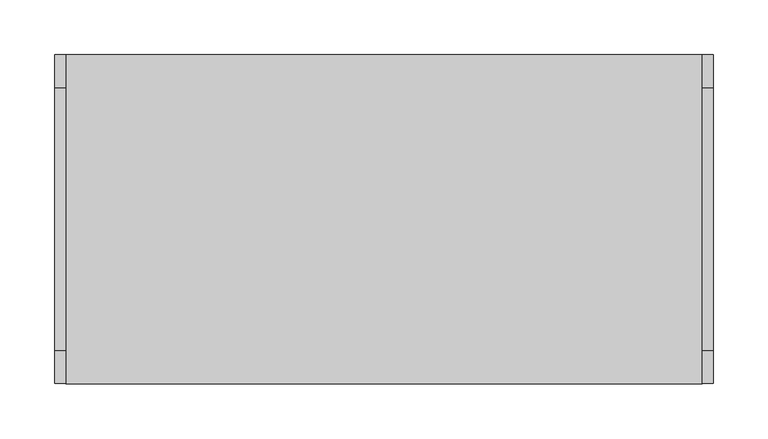
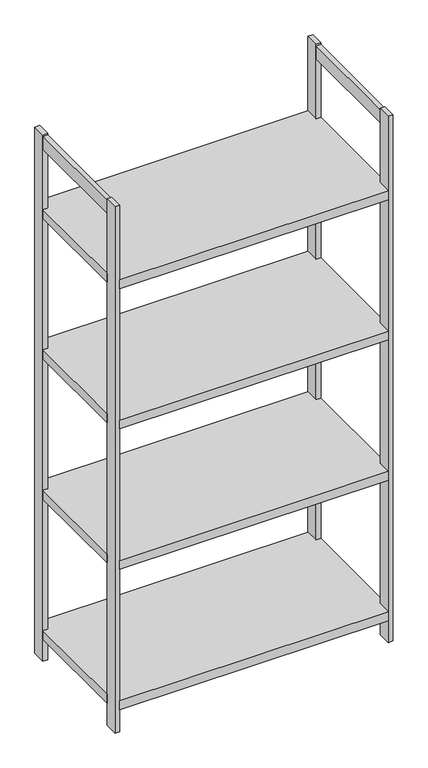
"""IFC4 building model written with IfcOpenShell, lengths in millimetres: furniture geometry, GEL-Shelf-一般オフィス棚 : GEL-Shelf-一般オフィス棚."""

import ifcopenshell
import ifcopenshell.guid

model = None  # the IFC model being written
_history = None  # IfcOwnerHistory: only IFC2X3 demands one
_inside = {}  # id of a spatial element -> (the spatial element, [elements in it])
_under = {}  # id of a project, library or spatial element -> (it, [spatial elements below it])
_declared = {}  # id of a project -> (the project, [libraries it declares])
_typed = {}  # id of a type object -> (the type object, [elements of that type])
_made_of = {}  # id of a material, layer set ... -> (it, [elements and type objects made of it])


def new_model(schema):
    """Start an empty IFC model of exactly this schema.

    Asked for "IFC4X3", IfcOpenShell would pick the latest addendum, in which some entities
    have other attributes; the version numbers below select the first issue.
    IFC2X3 requires an IfcOwnerHistory on every rooted entity: one is made here for all.
    """
    global model, _history
    if schema == "IFC4X3":
        model = ifcopenshell.file(schema_version=(4, 3, 0, 0))
    else:
        model = ifcopenshell.file(schema=schema)
    _inside.clear()
    _under.clear()
    _declared.clear()
    _typed.clear()
    _made_of.clear()
    _history = None
    if model.schema == "IFC2X3":
        org = make("IfcOrganization", Name="unknown")
        user = make(
            "IfcPersonAndOrganization",
            ThePerson=make("IfcPerson", FamilyName="unknown"),
            TheOrganization=org,
        )
        app = make(
            "IfcApplication",
            ApplicationDeveloper=org,
            Version="unknown",
            ApplicationFullName="unknown",
            ApplicationIdentifier="unknown",
        )
        _history = make(
            "IfcOwnerHistory",
            OwningUser=user,
            OwningApplication=app,
            ChangeAction="ADDED",
            CreationDate=0,
        )
    return model


def make(cls, **values):
    """One entity of the class cls with the attributes given. An attribute that is None is left unset."""
    return model.create_entity(
        cls, **{name: value for name, value in values.items() if value is not None}
    )


def rooted(cls, **values):
    """An entity with a GlobalId (a new one), such as an element, a storey or a relation."""
    return make(cls, GlobalId=ifcopenshell.guid.new(), OwnerHistory=_history, **values)


def si_unit(unit_type, name, prefix=None):
    """IfcSIUnit, for example si_unit("LENGTHUNIT", "METRE", prefix="MILLI")."""
    return make("IfcSIUnit", UnitType=unit_type, Prefix=prefix, Name=name)


def assignment(units):
    """IfcUnitAssignment: the units of a project."""
    return None if units is None else make("IfcUnitAssignment", Units=units)


def point(xyz):
    """IfcCartesianPoint."""
    return None if xyz is None else make("IfcCartesianPoint", Coordinates=xyz)


def direction(xyz):
    """IfcDirection."""
    return None if xyz is None else make("IfcDirection", DirectionRatios=xyz)


def frame(location, z_axis=None, x_axis=None):
    """IfcAxis2Placement3D, a coordinate frame: its origin and axes. An axis left out is left unset."""
    return make(
        "IfcAxis2Placement3D",
        Location=point(location),
        Axis=direction(z_axis),
        RefDirection=direction(x_axis),
    )


def origin():
    """The frame at (0, 0, 0) with its axes left unset."""
    return frame((0.0, 0.0, 0.0))


def origin_with_axes():
    """The frame at (0, 0, 0) with the z axis (0, 0, 1) and the x axis (1, 0, 0) written out."""
    return frame((0.0, 0.0, 0.0), z_axis=(0.0, 0.0, 1.0), x_axis=(1.0, 0.0, 0.0))


def place(relative_to, where):
    """IfcLocalPlacement: puts the frame where relative to a parent placement (None: the world)."""
    return make(
        "IfcLocalPlacement", PlacementRelTo=relative_to, RelativePlacement=where
    )


def context(
    kind, dimensions, precision=None, world=None, true_north=None, identifier=None
):
    """IfcGeometricRepresentationContext, for example the 3D "Model" context."""
    return make(
        "IfcGeometricRepresentationContext",
        ContextIdentifier=identifier,
        ContextType=kind,
        CoordinateSpaceDimension=dimensions,
        Precision=precision,
        WorldCoordinateSystem=world,
        TrueNorth=true_north,
    )


def project(units=None, contexts=None):
    """IfcProject with its units and contexts."""
    return rooted(
        "IfcProject",
        Name="project",
        RepresentationContexts=contexts,
        UnitsInContext=assignment(units),
    )


def spatial(cls, under=None, at=None, **own):
    """A site, building, storey or space (cls), placed at a placement, below another one or the project."""
    s = rooted(cls, ObjectPlacement=at, **own)
    if under is not None:
        _under.setdefault(under.id(), (under, []))[1].append(s)
    return s


def polyline(points):
    """IfcPolyline through the points."""
    return make("IfcPolyline", Points=[point(p) for p in points])


def outline(outer, holes=None, kind="AREA"):
    """IfcArbitraryClosedProfileDef: a profile drawn as a closed curve; with holes, ...WithVoids."""
    if holes is None:
        return make("IfcArbitraryClosedProfileDef", ProfileType=kind, OuterCurve=outer)
    return make(
        "IfcArbitraryProfileDefWithVoids",
        ProfileType=kind,
        OuterCurve=outer,
        InnerCurves=holes,
    )


def extrude(swept, where, along, depth):
    """IfcExtrudedAreaSolid: the profile swept, set in the frame where, extruded along a direction by depth."""
    return make(
        "IfcExtrudedAreaSolid",
        SweptArea=swept,
        Position=where,
        ExtrudedDirection=direction(along),
        Depth=depth,
    )


def shape(context_of_items, identifier, shape_type, items):
    """IfcShapeRepresentation: the items that make up one representation, for example the "Body"."""
    return make(
        "IfcShapeRepresentation",
        ContextOfItems=context_of_items,
        RepresentationIdentifier=identifier,
        RepresentationType=shape_type,
        Items=items,
    )


def source(mapping_origin, context_of_items, identifier, shape_type, items):
    """IfcRepresentationMap: a shape defined once, which mapped items show again and again."""
    return make(
        "IfcRepresentationMap",
        MappingOrigin=mapping_origin,
        MappedRepresentation=shape(context_of_items, identifier, shape_type, items),
    )


def transform(
    local_origin,
    x_axis=None,
    y_axis=None,
    z_axis=None,
    scale=None,
    scale2=None,
    scale3=None,
    uniform=True,
):
    """IfcCartesianTransformationOperator3D, or its non-uniform kind. x_axis, y_axis, z_axis: its Axis1, 2, 3."""
    if uniform:
        return make(
            "IfcCartesianTransformationOperator3D",
            Axis1=direction(x_axis),
            Axis2=direction(y_axis),
            LocalOrigin=point(local_origin),
            Scale=scale,
            Axis3=direction(z_axis),
        )
    return make(
        "IfcCartesianTransformationOperator3DnonUniform",
        Axis1=direction(x_axis),
        Axis2=direction(y_axis),
        LocalOrigin=point(local_origin),
        Scale=scale,
        Axis3=direction(z_axis),
        Scale2=scale2,
        Scale3=scale3,
    )


def mapped(mapping_source, mapping_target):
    """IfcMappedItem: shows the shape of a source again, moved by a transform."""
    return make(
        "IfcMappedItem", MappingSource=mapping_source, MappingTarget=mapping_target
    )


def made_of(thing, what):
    """Note that an element or type object is made of a material, layer set ...; save() writes the relation."""
    if what is not None:
        _made_of.setdefault(what.id(), (what, []))[1].append(thing)
    return thing


def element(
    cls,
    number,
    at=None,
    inside=None,
    cuts=None,
    type_object=None,
    material=None,
    context=None,
    identifier="Body",
    shape_type=None,
    held_by="IfcProductDefinitionShape",
    body=None,
    shapes=None,
    **own,
):
    """One element of the class cls, such as IfcWall. Its Tag is "e" and its number.

    at: its placement. inside: the storey or other place that contains it. cuts: it is an
    opening in that element (IfcRelVoidsElement). A single representation is given by context,
    identifier, shape_type and body (its items); several are given by shapes. held_by: the class
    of the entity that holds the representations. save() writes the other relations.
    """
    e = rooted(cls, Tag="e%d" % number, ObjectPlacement=at, **own)
    if body is not None:
        shapes = [shape(context, identifier, shape_type, body)]
    if shapes is not None:
        e.Representation = make(held_by, Representations=shapes)
    if inside is not None:
        _inside.setdefault(inside.id(), (inside, []))[1].append(e)
    if cuts is not None:
        rooted(
            "IfcRelVoidsElement", RelatingBuildingElement=cuts, RelatedOpeningElement=e
        )
    if type_object is not None:
        _typed.setdefault(type_object.id(), (type_object, []))[1].append(e)
    return made_of(e, material)


def aggregate(whole, parts):
    """IfcRelAggregates: a whole, such as a stair, and the parts it consists of."""
    return rooted("IfcRelAggregates", RelatingObject=whole, RelatedObjects=parts)


def save(model, path):
    """Write the relations noted so far, then the file.

    IfcRelAggregates (storeys below a building ...), IfcRelContainedInSpatialStructure (elements
    in a storey), IfcRelDefinesByType, IfcRelAssociatesMaterial and IfcRelDeclares: one each for
    every whole, place, type object, material and project.
    """
    for whole, parts in _under.values():
        aggregate(whole, parts)
    for where, things in _inside.values():
        rooted(
            "IfcRelContainedInSpatialStructure",
            RelatedElements=things,
            RelatingStructure=where,
        )
    for kind, things in _typed.values():
        rooted("IfcRelDefinesByType", RelatedObjects=things, RelatingType=kind)
    for what, things in _made_of.values():
        rooted("IfcRelAssociatesMaterial", RelatedObjects=things, RelatingMaterial=what)
    for by, libraries in _declared.values():
        rooted("IfcRelDeclares", RelatingContext=by, RelatedDefinitions=libraries)
    model.write(path)


def furniture_81dc58f3(model_context):
    return source(origin(), model_context, "Body", "SweptSolid", [
        extrude(outline(polyline([(300.0, -120.0), (290.0, -120.0), (290.0, -150.0), (-290.0, -150.0), (-290.0, -120.0), (-300.0, -120.0), (-300.0, 120.0), (-290.0, 120.0), (-290.0, 150.0), (290.0, 150.0), (290.0, 120.0), (300.0, 120.0), (300.0, -120.0)])), frame((0.0, 0.0, 50.0), z_axis=(0.0, 0.0, 1.0), x_axis=(1.0, 0.0, 0.0)), (0.0, 0.0, 1.0), 20.0),
        extrude(outline(polyline([(300.0, -120.0), (290.0, -120.0), (290.0, -150.0), (-290.0, -150.0), (-290.0, -120.0), (-300.0, -120.0), (-300.0, 120.0), (-290.0, 120.0), (-290.0, 150.0), (290.0, 150.0), (290.0, 120.0), (300.0, 120.0), (300.0, -120.0)])), frame((0.0, 0.0, 370.0), z_axis=(0.0, 0.0, 1.0), x_axis=(1.0, 0.0, 0.0)), (0.0, 0.0, 1.0), 20.0),
        extrude(outline(polyline([(300.0, -120.0), (290.0, -120.0), (290.0, -150.0), (-290.0, -150.0), (-290.0, -120.0), (-300.0, -120.0), (-300.0, 120.0), (-290.0, 120.0), (-290.0, 150.0), (290.0, 150.0), (290.0, 120.0), (300.0, 120.0), (300.0, -120.0)])), frame((0.0, 0.0, 690.0), z_axis=(0.0, 0.0, 1.0), x_axis=(1.0, 0.0, 0.0)), (0.0, 0.0, 1.0), 20.0),
        extrude(outline(polyline([(300.0, -120.0), (290.0, -120.0), (290.0, -150.0), (-290.0, -150.0), (-290.0, -120.0), (-300.0, -120.0), (-300.0, 120.0), (-290.0, 120.0), (-290.0, 150.0), (290.0, 150.0), (290.0, 120.0), (300.0, 120.0), (300.0, -120.0)])), frame((0.0, 0.0, 1010.0), z_axis=(0.0, 0.0, 1.0), x_axis=(1.0, 0.0, 0.0)), (0.0, 0.0, 1.0), 20.0),
        extrude(outline(polyline([(300.0, -150.0), (290.0, -150.0), (290.0, -120.0), (300.0, -120.0), (300.0, -150.0)])), origin_with_axes(), (0.0, 0.0, 1.0), 1200.0),
        extrude(outline(polyline([(300.0, 120.0), (290.0, 120.0), (290.0, 150.0), (300.0, 150.0), (300.0, 120.0)])), origin_with_axes(), (0.0, 0.0, 1.0), 1200.0),
        extrude(outline(polyline([(-290.0, 120.0), (-300.0, 120.0), (-300.0, 150.0), (-290.0, 150.0), (-290.0, 120.0)])), origin_with_axes(), (0.0, 0.0, 1.0), 1200.0),
        extrude(outline(polyline([(-290.0, -150.0), (-300.0, -150.0), (-300.0, -120.0), (-290.0, -120.0), (-290.0, -150.0)])), origin_with_axes(), (0.0, 0.0, 1.0), 1200.0),
        extrude(outline(polyline([(-290.0, -120.0), (-300.0, -120.0), (-300.0, 120.0), (-290.0, 120.0), (-290.0, -120.0)])), frame((0.0, 0.0, 1167.0), z_axis=(0.0, 0.0, 1.0), x_axis=(1.0, 0.0, 0.0)), (0.0, 0.0, 1.0), 30.0),
        extrude(outline(polyline([(300.0, -120.0), (290.0, -120.0), (290.0, 120.0), (300.0, 120.0), (300.0, -120.0)])), frame((0.0, 0.0, 1167.0), z_axis=(0.0, 0.0, 1.0), x_axis=(1.0, 0.0, 0.0)), (0.0, 0.0, 1.0), 30.0),
    ])


if __name__ == "__main__":
    model = new_model("IFC4")
    model_context = context("Model", 3, world=origin())
    ifc_project = project(units=[si_unit("LENGTHUNIT", "METRE", prefix="MILLI")], contexts=[model_context])
    site = spatial("IfcSite", under=ifc_project)
    building = spatial("IfcBuilding", under=site)
    placement = place(None, origin())
    furniture_shape = furniture_81dc58f3(model_context)
    element("IfcFurniture", 1, ObjectType="GEL-Shelf-一般オフィス棚 : GEL-Shelf-一般オフィス棚", at=placement, inside=building, context=model_context, shape_type="MappedRepresentation", body=[
        mapped(furniture_shape, transform((0.0, 0.0, 0.0), x_axis=(1.0, 0.0, 0.0), y_axis=(0.0, 1.0, 0.0), z_axis=(0.0, 0.0, 1.0))),
    ])
    save(model, "model.ifc")

# Revit data of these elements
# Project information
#   プロジェクト発行日 = "発行日"
#   プロジェクト ステータス = "プロジェクト ステータス"
#   クライアント名 = "オーナ"
#   計画地住所 = "ここにアドレスを入力"
#   プロジェクト名 = "プロジェクト名"
#   プロジェクト番号 = "0001"
# Type "GEL-Shelf-一般オフィス棚 : GEL-Shelf-一般オフィス棚"
#   GEL-Width = 600 mm
#   GEL-Height = 1200 mm
#   GEL-Depth = 300 mm
#   GEL-Material-Support = Black Opaque Plastic
#   GEL-Material-Shelf = Iroko polished
#   GEL-Material-Base = none
#   GEL-Material-Accent = none
#   Default Elevation = 0
# Element 1 (IfcFurniture, "GEL-Shelf-一般オフィス棚 : GEL-Shelf-一般オフィス棚")
#   Materials on its faces: "Iroko polished", "Black Opaque Plastic"
# Materials
#   "Black Opaque Plastic": class "一般", colour RGB 0 0 0, transparency 0, Cost = 0
#   "Iroko polished": class "一般", colour RGB 156 100 46, transparency 0, Cost = 0
